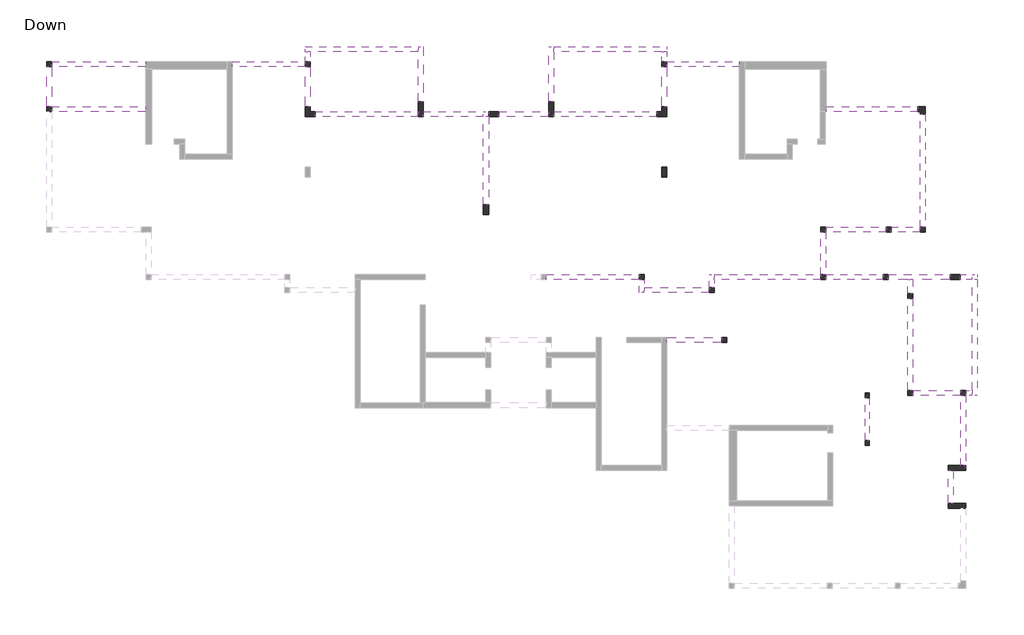
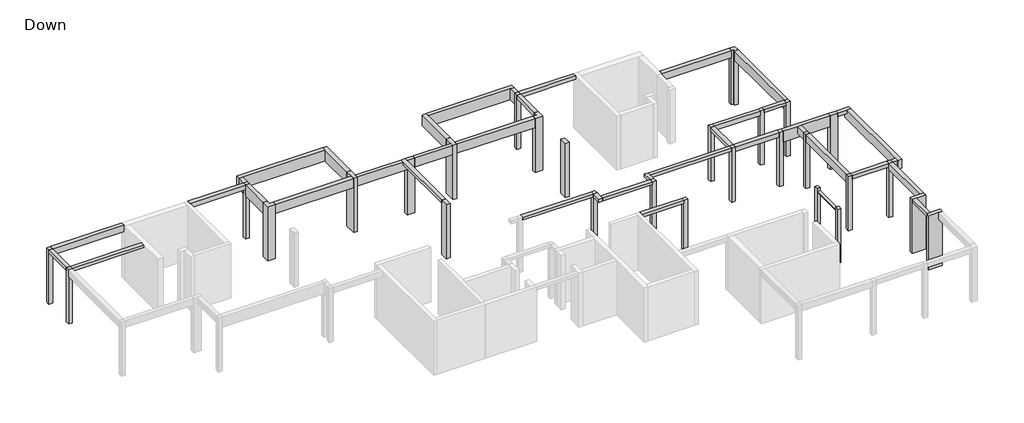
# One storey, part 2 of 2: 40 beams, 28 columns.
# Revit data of these elements (continued)
# Element 24 (IfcBeam, "Concrete Rectengular Beam : 20/40") (continued)
#   Comments = ""
#   Mark = "B40"
#   SOFiSTiK_AMG_Comments = ""
#   SOFiSTiK_AMG_Scheduled = yes
#   SOFiSTiK_AMG_Adjusted = yes
#   Structural Material = Concrete
#   Phase Created = New Construction
#   Materials on its faces: "Concrete"
# Element 25 (IfcBeam, "Concrete Rectengular Beam : 20/40")
#   Comments = ""
#   Mark = "B41"
#   SOFiSTiK_AMG_Comments = ""
#   SOFiSTiK_AMG_Scheduled = yes
#   SOFiSTiK_AMG_Adjusted = yes
#   Structural Material = Concrete
#   Phase Created = New Construction
#   Materials on its faces: "Concrete"
# Element 26 (IfcBeam, "Concrete Rectengular Beam : 20/40")
#   Comments = ""
#   Mark = "B42"
#   SOFiSTiK_AMG_Comments = ""
#   SOFiSTiK_AMG_Scheduled = yes
#   SOFiSTiK_AMG_Adjusted = yes
#   Structural Material = Concrete
#   Phase Created = New Construction
#   Materials on its faces: "Concrete"
# Element 27 (IfcBeam, "Concrete Rectengular Beam : 20/50")
#   Comments = ""
#   Mark = "B44"
#   SOFiSTiK_AMG_Comments = ""
#   SOFiSTiK_AMG_Scheduled = yes
#   SOFiSTiK_AMG_Adjusted = yes
#   Structural Material = Concrete
#   Phase Created = New Construction
#   Materials on its faces: "Concrete"
# Element 28 (IfcBeam, "Concrete Rectengular Beam : 20/50")
#   Comments = ""
#   Mark = "B45"
#   SOFiSTiK_AMG_Comments = ""
#   SOFiSTiK_AMG_Scheduled = yes
#   SOFiSTiK_AMG_Adjusted = yes
#   Structural Material = Concrete
#   Phase Created = New Construction
#   Materials on its faces: "Concrete"
# Element 29 (IfcBeam, "Concrete Rectengular Beam : 20/50")
#   Comments = ""
#   Mark = "B46"
#   SOFiSTiK_AMG_Comments = ""
#   SOFiSTiK_AMG_Scheduled = yes
#   SOFiSTiK_AMG_Adjusted = yes
#   Structural Material = Concrete
#   Phase Created = New Construction
#   Materials on its faces: "Concrete"
# Element 30 (IfcBeam, "Concrete Rectengular Beam : 20/50")
#   Comments = ""
#   Mark = "B47"
#   SOFiSTiK_AMG_Comments = ""
#   SOFiSTiK_AMG_Scheduled = yes
#   SOFiSTiK_AMG_Adjusted = yes
#   Structural Material = Concrete
#   Phase Created = New Construction
#   Materials on its faces: "Concrete"
# Element 31 (IfcBeam, "Concrete Rectengular Beam : 20/50")
#   Comments = ""
#   Mark = "B48"
#   SOFiSTiK_AMG_Comments = ""
#   SOFiSTiK_AMG_Scheduled = yes
#   SOFiSTiK_AMG_Adjusted = yes
#   Structural Material = Concrete
#   Phase Created = New Construction
#   Materials on its faces: "Concrete"
# Element 32 (IfcBeam, "Concrete Rectengular Beam : 20/50")
#   Comments = ""
#   Mark = "B49"
#   SOFiSTiK_AMG_Comments = ""
#   SOFiSTiK_AMG_Scheduled = yes
#   SOFiSTiK_AMG_Adjusted = yes
#   Structural Material = Concrete
#   Phase Created = New Construction
#   Materials on its faces: "Concrete"
# Element 33 (IfcBeam, "Concrete Rectengular Beam : 20/60")
#   Comments = ""
#   Mark = "B50"
#   SOFiSTiK_AMG_Comments = ""
#   SOFiSTiK_AMG_Scheduled = yes
#   SOFiSTiK_AMG_Adjusted = yes
#   Structural Material = Concrete
#   Phase Created = New Construction
#   Materials on its faces: "Concrete"
# Element 34 (IfcBeam, "Concrete Rectengular Beam : 20/60")
#   Comments = ""
#   Mark = "B51"
#   SOFiSTiK_AMG_Comments = ""
#   SOFiSTiK_AMG_Scheduled = yes
#   SOFiSTiK_AMG_Adjusted = yes
#   Structural Material = Concrete
#   Phase Created = New Construction
#   Materials on its faces: "Concrete"
# Element 35 (IfcBeam, "Concrete Rectengular Beam : 20/60")
#   Comments = ""
#   Mark = "B52"
#   SOFiSTiK_AMG_Comments = ""
#   SOFiSTiK_AMG_Scheduled = yes
#   SOFiSTiK_AMG_Adjusted = yes
#   Structural Material = Concrete
#   Phase Created = New Construction
#   Materials on its faces: "Concrete"
# Element 36 (IfcBeam, "Concrete Rectengular Beam : 20/60")
#   Comments = ""
#   Mark = "B53"
#   SOFiSTiK_AMG_Comments = ""
#   SOFiSTiK_AMG_Scheduled = yes
#   SOFiSTiK_AMG_Adjusted = yes
#   Structural Material = Concrete
#   Phase Created = New Construction
#   Materials on its faces: "Concrete"
# Element 37 (IfcBeam, "Concrete Rectengular Beam : 20/60")
#   Comments = ""
#   Mark = "B54"
#   SOFiSTiK_AMG_Comments = ""
#   SOFiSTiK_AMG_Scheduled = yes
#   SOFiSTiK_AMG_Adjusted = yes
#   Structural Material = Concrete
#   Phase Created = New Construction
#   Materials on its faces: "Concrete"
# Element 38 (IfcBeam, "Concrete Rectengular Beam : 20/60")
#   Comments = ""
#   Mark = "B55"
#   SOFiSTiK_AMG_Comments = ""
#   SOFiSTiK_AMG_Scheduled = yes
#   SOFiSTiK_AMG_Adjusted = yes
#   Structural Material = Concrete
#   Phase Created = New Construction
#   Materials on its faces: "Concrete"
# Element 39 (IfcBeam, "Concrete Rectengular Beam : 20/60")
#   Comments = ""
#   Mark = "B56"
#   SOFiSTiK_AMG_Comments = ""
#   SOFiSTiK_AMG_Scheduled = yes
#   SOFiSTiK_AMG_Adjusted = yes
#   Structural Material = Concrete
#   Phase Created = New Construction
#   Materials on its faces: "Concrete"
# Element 40 (IfcBeam, "Concrete Rectengular Beam : 20/60")
#   Comments = ""
#   Mark = "B59"
#   SOFiSTiK_AMG_Comments = ""
#   SOFiSTiK_AMG_Scheduled = yes
#   SOFiSTiK_AMG_Adjusted = yes
#   Structural Material = Concrete
#   Phase Created = New Construction
#   Materials on its faces: "Concrete"
# Element 41 (IfcColumn, "Concrete Rectengular Column : 16/20")
#   Comments = ""
#   Mark = "C1"
#   SOFiSTiK_AMG_Comments = ""
#   SOFiSTiK_AMG_Scheduled = yes
#   SOFiSTiK_AMG_Adjusted = yes
#   Structural Material = Concrete
#   Phase Created = New Construction
#   Materials on its faces: "Concrete"
# Element 42 (IfcColumn, "Concrete Rectengular Column : 16/20")
#   Comments = ""
#   Mark = "C2"
#   SOFiSTiK_AMG_Comments = ""
#   SOFiSTiK_AMG_Scheduled = yes
#   SOFiSTiK_AMG_Adjusted = yes
#   Structural Material = Concrete
#   Phase Created = New Construction
#   Materials on its faces: "Concrete"
# Element 43 (IfcColumn, "Concrete Rectengular Column : 20/20")
#   Comments = ""
#   Mark = "C6"
#   SOFiSTiK_AMG_Comments = ""
#   SOFiSTiK_AMG_Scheduled = yes
#   SOFiSTiK_AMG_Adjusted = yes
#   Structural Material = Concrete
#   Phase Created = New Construction
#   Materials on its faces: "Concrete"
# Element 44 (IfcColumn, "Concrete Rectengular Column : 20/20")
#   Comments = ""
#   Mark = "C7"
#   SOFiSTiK_AMG_Comments = ""
#   SOFiSTiK_AMG_Scheduled = yes
#   SOFiSTiK_AMG_Adjusted = yes
#   Structural Material = Concrete
#   Phase Created = New Construction
#   Materials on its faces: "Concrete"
# Element 45 (IfcColumn, "Concrete Rectengular Column : 20/20")
#   Comments = ""
#   Mark = "C8"
#   SOFiSTiK_AMG_Comments = ""
#   SOFiSTiK_AMG_Scheduled = yes
#   SOFiSTiK_AMG_Adjusted = yes
#   Structural Material = Concrete
#   Phase Created = New Construction
#   Materials on its faces: "Concrete"
# Element 46 (IfcColumn, "Concrete Rectengular Column : 20/20")
#   Comments = ""
#   Mark = "C9"
#   SOFiSTiK_AMG_Comments = ""
#   SOFiSTiK_AMG_Scheduled = yes
#   SOFiSTiK_AMG_Adjusted = yes
#   Structural Material = Concrete
#   Phase Created = New Construction
#   Materials on its faces: "Concrete"
# Element 47 (IfcColumn, "Concrete Rectengular Column : 20/20")
#   Comments = ""
#   Mark = "C10"
#   SOFiSTiK_AMG_Comments = ""
#   SOFiSTiK_AMG_Scheduled = yes
#   SOFiSTiK_AMG_Adjusted = yes
#   Structural Material = Concrete
#   Phase Created = New Construction
#   Materials on its faces: "Concrete"
# Element 48 (IfcColumn, "Concrete Rectengular Column : 20/20")
#   Comments = ""
#   Mark = "C11"
#   SOFiSTiK_AMG_Comments = ""
#   SOFiSTiK_AMG_Scheduled = yes
#   SOFiSTiK_AMG_Adjusted = yes
#   Structural Material = Concrete
#   Phase Created = New Construction
#   Materials on its faces: "Concrete"
# Element 49 (IfcColumn, "Concrete Rectengular Column : 20/20")
#   Comments = ""
#   Mark = "C12"
#   SOFiSTiK_AMG_Comments = ""
#   SOFiSTiK_AMG_Scheduled = yes
#   SOFiSTiK_AMG_Adjusted = yes
#   Structural Material = Concrete
#   Phase Created = New Construction
#   Materials on its faces: "Concrete"
# Element 50 (IfcColumn, "Concrete Rectengular Column : 20/20")
#   Comments = ""
#   Mark = "C16"
#   SOFiSTiK_AMG_Comments = ""
#   SOFiSTiK_AMG_Scheduled = yes
#   SOFiSTiK_AMG_Adjusted = yes
#   Structural Material = Concrete
#   Phase Created = New Construction
#   Materials on its faces: "Concrete"
# Element 51 (IfcColumn, "Concrete Rectengular Column : 20/20")
#   Comments = ""
#   Mark = "C17"
#   SOFiSTiK_AMG_Comments = ""
#   SOFiSTiK_AMG_Scheduled = yes
#   SOFiSTiK_AMG_Adjusted = yes
#   Structural Material = Concrete
#   Phase Created = New Construction
#   Materials on its faces: "Concrete"
# Element 52 (IfcColumn, "Concrete Rectengular Column : 20/20")
#   Comments = ""
#   Mark = "C18"
#   SOFiSTiK_AMG_Comments = ""
#   SOFiSTiK_AMG_Scheduled = yes
#   SOFiSTiK_AMG_Adjusted = yes
#   Structural Material = Concrete
#   Phase Created = New Construction
#   Materials on its faces: "Concrete"
# Element 53 (IfcColumn, "Concrete Rectengular Column : 20/20")
#   Comments = ""
#   Mark = "C19"
#   SOFiSTiK_AMG_Comments = ""
#   SOFiSTiK_AMG_Scheduled = yes
#   SOFiSTiK_AMG_Adjusted = yes
#   Structural Material = Concrete
#   Phase Created = New Construction
#   Materials on its faces: "Concrete"
# Element 54 (IfcColumn, "Concrete Rectengular Column : 20/20")
#   Comments = ""
#   Mark = "C20"
#   SOFiSTiK_AMG_Comments = ""
#   SOFiSTiK_AMG_Scheduled = yes
#   SOFiSTiK_AMG_Adjusted = yes
#   Structural Material = Concrete
#   Phase Created = New Construction
#   Materials on its faces: "Concrete"
# Element 55 (IfcColumn, "Concrete Rectengular Column : 20/20")
#   Comments = ""
#   Mark = "C21"
#   SOFiSTiK_AMG_Comments = ""
#   SOFiSTiK_AMG_Scheduled = yes
#   SOFiSTiK_AMG_Adjusted = yes
#   Structural Material = Concrete
#   Phase Created = New Construction
#   Materials on its faces: "Concrete"
# Element 56 (IfcColumn, "Concrete Rectengular Column : 20/20")
#   Comments = ""
#   Mark = "C22"
#   SOFiSTiK_AMG_Comments = ""
#   SOFiSTiK_AMG_Scheduled = yes
#   SOFiSTiK_AMG_Adjusted = yes
#   Structural Material = Concrete
#   Phase Created = New Construction
#   Materials on its faces: "Concrete"
# Element 57 (IfcColumn, "Concrete Rectengular Column : 20/20")
#   Comments = ""
#   Mark = "C23"
#   SOFiSTiK_AMG_Comments = ""
#   SOFiSTiK_AMG_Scheduled = yes
#   SOFiSTiK_AMG_Adjusted = yes
#   Structural Material = Concrete
#   Phase Created = New Construction
#   Materials on its faces: "Concrete"
# Element 58 (IfcColumn, "Concrete Rectengular Column : 20/40")
#   Comments = ""
#   Mark = "C28"
#   SOFiSTiK_AMG_Comments = ""
#   SOFiSTiK_AMG_Scheduled = yes
#   SOFiSTiK_AMG_Adjusted = yes
#   Structural Material = Concrete
#   Phase Created = New Construction
#   Materials on its faces: "Concrete"
# Element 59 (IfcColumn, "Concrete Rectengular Column : 20/40")
#   Comments = ""
#   Mark = "C29"
#   SOFiSTiK_AMG_Comments = ""
#   SOFiSTiK_AMG_Scheduled = yes
#   SOFiSTiK_AMG_Adjusted = yes
#   Structural Material = Concrete
#   Phase Created = New Construction
#   Materials on its faces: "Concrete"
# Element 60 (IfcColumn, "Concrete Rectengular Column : 20/40")
#   Comments = ""
#   Mark = "C30"
#   SOFiSTiK_AMG_Comments = ""
#   SOFiSTiK_AMG_Scheduled = yes
#   SOFiSTiK_AMG_Adjusted = yes
#   Structural Material = Concrete
#   Phase Created = New Construction
#   Materials on its faces: "Concrete"
# Element 61 (IfcColumn, "Concrete Rectengular Column : 20/40")
#   Comments = ""
#   Mark = "C33"
#   SOFiSTiK_AMG_Comments = ""
#   SOFiSTiK_AMG_Scheduled = yes
#   SOFiSTiK_AMG_Adjusted = yes
#   Structural Material = Concrete
#   Phase Created = New Construction
#   Materials on its faces: "Concrete"
# Element 62 (IfcColumn, "Concrete Rectengular Column : 20/60")
#   Comments = ""
#   Mark = "C34"
#   SOFiSTiK_AMG_Comments = ""
#   SOFiSTiK_AMG_Scheduled = yes
#   SOFiSTiK_AMG_Adjusted = yes
#   Structural Material = Concrete
#   Phase Created = New Construction
#   Materials on its faces: "Concrete"
# Element 63 (IfcColumn, "Concrete Rectengular Column : 20/60")
#   Comments = ""
#   Mark = "C35"
#   SOFiSTiK_AMG_Comments = ""
#   SOFiSTiK_AMG_Scheduled = yes
#   SOFiSTiK_AMG_Adjusted = yes
#   Structural Material = Concrete
#   Phase Created = New Construction
#   Materials on its faces: "Concrete"
# Element 64 (IfcColumn, "Concrete Rectengular Column : 20/70")
#   Comments = ""
#   Mark = "C36"
#   SOFiSTiK_AMG_Comments = ""
#   SOFiSTiK_AMG_Scheduled = yes
#   SOFiSTiK_AMG_Adjusted = yes
#   Structural Material = Concrete
#   Phase Created = New Construction
#   Materials on its faces: "Concrete"
# Element 65 (IfcColumn, "Concrete Rectengular Column : 20/70")
#   Comments = ""
#   Mark = "C37"
#   SOFiSTiK_AMG_Comments = ""
#   SOFiSTiK_AMG_Scheduled = yes
#   SOFiSTiK_AMG_Adjusted = yes
#   Structural Material = Concrete
#   Phase Created = New Construction
#   Materials on its faces: "Concrete"
# Element 66 (IfcColumn, "L Column : 30/30/20/20")
#   Comments = ""
#   Mark = "C39"
#   SOFiSTiK_AMG_Comments = ""
#   SOFiSTiK_AMG_Scheduled = yes
#   SOFiSTiK_AMG_Adjusted = yes
#   Structural Material = Concrete
#   Phase Created = New Construction
# Element 67 (IfcColumn, "L Column : 40/40/20/20")
#   Comments = ""
#   Mark = "C40"
#   SOFiSTiK_AMG_Comments = ""
#   SOFiSTiK_AMG_Scheduled = yes
#   SOFiSTiK_AMG_Adjusted = yes
#   Structural Material = Concrete
#   Phase Created = New Construction
# Element 68 (IfcColumn, "L Column : 40/40/20/20")
#   Comments = ""
#   Mark = "C41"
#   SOFiSTiK_AMG_Comments = ""
#   SOFiSTiK_AMG_Scheduled = yes
#   SOFiSTiK_AMG_Adjusted = yes
#   Structural Material = Concrete
#   Phase Created = New Construction
# Materials
#   "Concrete": class "Concrete", colour RGB 192 192 192, transparency 0, Keynote = "01000", Description = "Cast-in-place concrete", Cost = 0
#   "Concrete, Cast-in-Place gray": class "Concrete", colour RGB 192 192 192, transparency 0, Description = "Cast-in-place concrete", Cost = 0
